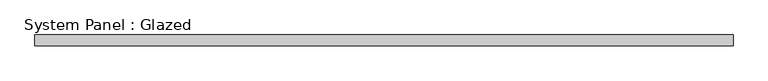
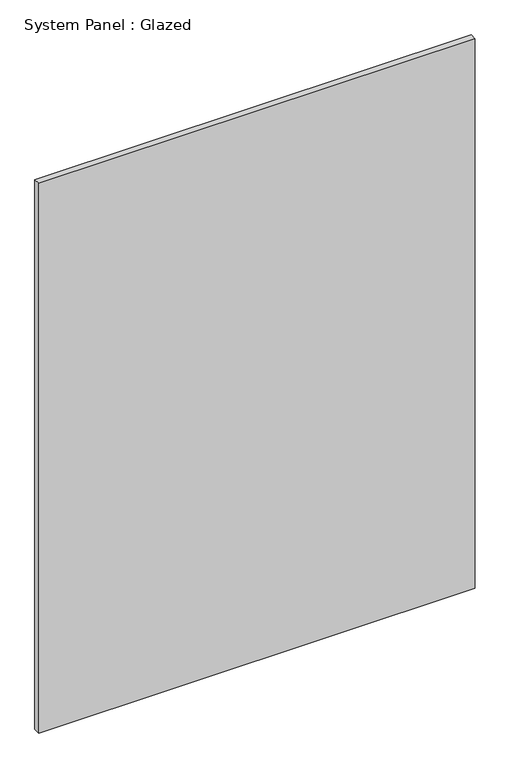
"""IFC4 building model written with IfcOpenShell, lengths in millimetres: plate geometry, System Panel : Glazed."""

import ifcopenshell
import ifcopenshell.guid

model = None  # the IFC model being written
_history = None  # IfcOwnerHistory: only IFC2X3 demands one
_inside = {}  # id of a spatial element -> (the spatial element, [elements in it])
_under = {}  # id of a project, library or spatial element -> (it, [spatial elements below it])
_declared = {}  # id of a project -> (the project, [libraries it declares])
_typed = {}  # id of a type object -> (the type object, [elements of that type])
_made_of = {}  # id of a material, layer set ... -> (it, [elements and type objects made of it])


def new_model(schema):
    """Start an empty IFC model of exactly this schema.

    Asked for "IFC4X3", IfcOpenShell would pick the latest addendum, in which some entities
    have other attributes; the version numbers below select the first issue.
    IFC2X3 requires an IfcOwnerHistory on every rooted entity: one is made here for all.
    """
    global model, _history
    if schema == "IFC4X3":
        model = ifcopenshell.file(schema_version=(4, 3, 0, 0))
    else:
        model = ifcopenshell.file(schema=schema)
    _inside.clear()
    _under.clear()
    _declared.clear()
    _typed.clear()
    _made_of.clear()
    _history = None
    if model.schema == "IFC2X3":
        org = make("IfcOrganization", Name="unknown")
        user = make(
            "IfcPersonAndOrganization",
            ThePerson=make("IfcPerson", FamilyName="unknown"),
            TheOrganization=org,
        )
        app = make(
            "IfcApplication",
            ApplicationDeveloper=org,
            Version="unknown",
            ApplicationFullName="unknown",
            ApplicationIdentifier="unknown",
        )
        _history = make(
            "IfcOwnerHistory",
            OwningUser=user,
            OwningApplication=app,
            ChangeAction="ADDED",
            CreationDate=0,
        )
    return model


def make(cls, **values):
    """One entity of the class cls with the attributes given. An attribute that is None is left unset."""
    return model.create_entity(
        cls, **{name: value for name, value in values.items() if value is not None}
    )


def rooted(cls, **values):
    """An entity with a GlobalId (a new one), such as an element, a storey or a relation."""
    return make(cls, GlobalId=ifcopenshell.guid.new(), OwnerHistory=_history, **values)


def si_unit(unit_type, name, prefix=None):
    """IfcSIUnit, for example si_unit("LENGTHUNIT", "METRE", prefix="MILLI")."""
    return make("IfcSIUnit", UnitType=unit_type, Prefix=prefix, Name=name)


def assignment(units):
    """IfcUnitAssignment: the units of a project."""
    return None if units is None else make("IfcUnitAssignment", Units=units)


def point(xyz):
    """IfcCartesianPoint."""
    return None if xyz is None else make("IfcCartesianPoint", Coordinates=xyz)


def direction(xyz):
    """IfcDirection."""
    return None if xyz is None else make("IfcDirection", DirectionRatios=xyz)


def frame(location, z_axis=None, x_axis=None):
    """IfcAxis2Placement3D, a coordinate frame: its origin and axes. An axis left out is left unset."""
    return make(
        "IfcAxis2Placement3D",
        Location=point(location),
        Axis=direction(z_axis),
        RefDirection=direction(x_axis),
    )


def origin():
    """The frame at (0, 0, 0) with its axes left unset."""
    return frame((0.0, 0.0, 0.0))


def origin_with_axes():
    """The frame at (0, 0, 0) with the z axis (0, 0, 1) and the x axis (1, 0, 0) written out."""
    return frame((0.0, 0.0, 0.0), z_axis=(0.0, 0.0, 1.0), x_axis=(1.0, 0.0, 0.0))


def place(relative_to, where):
    """IfcLocalPlacement: puts the frame where relative to a parent placement (None: the world)."""
    return make(
        "IfcLocalPlacement", PlacementRelTo=relative_to, RelativePlacement=where
    )


def context(
    kind, dimensions, precision=None, world=None, true_north=None, identifier=None
):
    """IfcGeometricRepresentationContext, for example the 3D "Model" context."""
    return make(
        "IfcGeometricRepresentationContext",
        ContextIdentifier=identifier,
        ContextType=kind,
        CoordinateSpaceDimension=dimensions,
        Precision=precision,
        WorldCoordinateSystem=world,
        TrueNorth=true_north,
    )


def project(units=None, contexts=None):
    """IfcProject with its units and contexts."""
    return rooted(
        "IfcProject",
        Name="project",
        RepresentationContexts=contexts,
        UnitsInContext=assignment(units),
    )


def spatial(cls, under=None, at=None, **own):
    """A site, building, storey or space (cls), placed at a placement, below another one or the project."""
    s = rooted(cls, ObjectPlacement=at, **own)
    if under is not None:
        _under.setdefault(under.id(), (under, []))[1].append(s)
    return s


def polyline(points):
    """IfcPolyline through the points."""
    return make("IfcPolyline", Points=[point(p) for p in points])


def outline(outer, holes=None, kind="AREA"):
    """IfcArbitraryClosedProfileDef: a profile drawn as a closed curve; with holes, ...WithVoids."""
    if holes is None:
        return make("IfcArbitraryClosedProfileDef", ProfileType=kind, OuterCurve=outer)
    return make(
        "IfcArbitraryProfileDefWithVoids",
        ProfileType=kind,
        OuterCurve=outer,
        InnerCurves=holes,
    )


def extrude(swept, where, along, depth):
    """IfcExtrudedAreaSolid: the profile swept, set in the frame where, extruded along a direction by depth."""
    return make(
        "IfcExtrudedAreaSolid",
        SweptArea=swept,
        Position=where,
        ExtrudedDirection=direction(along),
        Depth=depth,
    )


def shape(context_of_items, identifier, shape_type, items):
    """IfcShapeRepresentation: the items that make up one representation, for example the "Body"."""
    return make(
        "IfcShapeRepresentation",
        ContextOfItems=context_of_items,
        RepresentationIdentifier=identifier,
        RepresentationType=shape_type,
        Items=items,
    )


def source(mapping_origin, context_of_items, identifier, shape_type, items):
    """IfcRepresentationMap: a shape defined once, which mapped items show again and again."""
    return make(
        "IfcRepresentationMap",
        MappingOrigin=mapping_origin,
        MappedRepresentation=shape(context_of_items, identifier, shape_type, items),
    )


def transform(
    local_origin,
    x_axis=None,
    y_axis=None,
    z_axis=None,
    scale=None,
    scale2=None,
    scale3=None,
    uniform=True,
):
    """IfcCartesianTransformationOperator3D, or its non-uniform kind. x_axis, y_axis, z_axis: its Axis1, 2, 3."""
    if uniform:
        return make(
            "IfcCartesianTransformationOperator3D",
            Axis1=direction(x_axis),
            Axis2=direction(y_axis),
            LocalOrigin=point(local_origin),
            Scale=scale,
            Axis3=direction(z_axis),
        )
    return make(
        "IfcCartesianTransformationOperator3DnonUniform",
        Axis1=direction(x_axis),
        Axis2=direction(y_axis),
        LocalOrigin=point(local_origin),
        Scale=scale,
        Axis3=direction(z_axis),
        Scale2=scale2,
        Scale3=scale3,
    )


def mapped(mapping_source, mapping_target):
    """IfcMappedItem: shows the shape of a source again, moved by a transform."""
    return make(
        "IfcMappedItem", MappingSource=mapping_source, MappingTarget=mapping_target
    )


def made_of(thing, what):
    """Note that an element or type object is made of a material, layer set ...; save() writes the relation."""
    if what is not None:
        _made_of.setdefault(what.id(), (what, []))[1].append(thing)
    return thing


def element(
    cls,
    number,
    at=None,
    inside=None,
    cuts=None,
    type_object=None,
    material=None,
    context=None,
    identifier="Body",
    shape_type=None,
    held_by="IfcProductDefinitionShape",
    body=None,
    shapes=None,
    **own,
):
    """One element of the class cls, such as IfcWall. Its Tag is "e" and its number.

    at: its placement. inside: the storey or other place that contains it. cuts: it is an
    opening in that element (IfcRelVoidsElement). A single representation is given by context,
    identifier, shape_type and body (its items); several are given by shapes. held_by: the class
    of the entity that holds the representations. save() writes the other relations.
    """
    e = rooted(cls, Tag="e%d" % number, ObjectPlacement=at, **own)
    if body is not None:
        shapes = [shape(context, identifier, shape_type, body)]
    if shapes is not None:
        e.Representation = make(held_by, Representations=shapes)
    if inside is not None:
        _inside.setdefault(inside.id(), (inside, []))[1].append(e)
    if cuts is not None:
        rooted(
            "IfcRelVoidsElement", RelatingBuildingElement=cuts, RelatedOpeningElement=e
        )
    if type_object is not None:
        _typed.setdefault(type_object.id(), (type_object, []))[1].append(e)
    return made_of(e, material)


def aggregate(whole, parts):
    """IfcRelAggregates: a whole, such as a stair, and the parts it consists of."""
    return rooted("IfcRelAggregates", RelatingObject=whole, RelatedObjects=parts)


def save(model, path):
    """Write the relations noted so far, then the file.

    IfcRelAggregates (storeys below a building ...), IfcRelContainedInSpatialStructure (elements
    in a storey), IfcRelDefinesByType, IfcRelAssociatesMaterial and IfcRelDeclares: one each for
    every whole, place, type object, material and project.
    """
    for whole, parts in _under.values():
        aggregate(whole, parts)
    for where, things in _inside.values():
        rooted(
            "IfcRelContainedInSpatialStructure",
            RelatedElements=things,
            RelatingStructure=where,
        )
    for kind, things in _typed.values():
        rooted("IfcRelDefinesByType", RelatedObjects=things, RelatingType=kind)
    for what, things in _made_of.values():
        rooted("IfcRelAssociatesMaterial", RelatedObjects=things, RelatingMaterial=what)
    for by, libraries in _declared.values():
        rooted("IfcRelDeclares", RelatingContext=by, RelatedDefinitions=libraries)
    model.write(path)


def system_panel_glazed_3d35191a(model_context):
    return source(origin(), model_context, "Body", "SweptSolid", [
        extrude(outline(polyline([(807.775, -49.5), (-807.775, -49.5), (-807.775, -24.5), (807.775, -24.5), (807.775, -49.5)])), origin_with_axes(), (0.0, 0.0, 1.0), 2150.0),
    ])


if __name__ == "__main__":
    model = new_model("IFC4")
    model_context = context("Model", 3, world=origin())
    ifc_project = project(units=[si_unit("LENGTHUNIT", "METRE", prefix="MILLI")], contexts=[model_context])
    site = spatial("IfcSite", under=ifc_project)
    building = spatial("IfcBuilding", under=site)
    placement = place(None, origin())
    system_panel_glazed_shape = system_panel_glazed_3d35191a(model_context)
    element("IfcPlate", 1, ObjectType="System Panel : Glazed", at=placement, inside=building, context=model_context, shape_type="MappedRepresentation", body=[
        mapped(system_panel_glazed_shape, transform((0.0, 0.0, 0.0), x_axis=(1.0, 0.0, 0.0), y_axis=(0.0, 1.0, 0.0), z_axis=(0.0, 0.0, 1.0))),
    ])
    save(model, "model.ifc")

# Revit data of these elements
# Type "System Panel : Glazed"
#   Keynote = "H11"
#   Construction Type Id = "GSP4R"
#   Analytic Construction = "1/8 in Pilkington single glazing"
#   Visual Light Transmittance = 0.9
#   Solar Heat Gain Coefficient = 0.86
#   Heat Transfer Coefficient (U) = 6.7069 W/(m²·K)
# Element 1 (IfcPlate, "System Panel : Glazed")
#   Materials on its faces: "Glass"
# Materials
#   "Glass": class "Glass", colour RGB 0 128 192, transparency 0.9, Description = "Soda Lime Glass", Cost = 0
